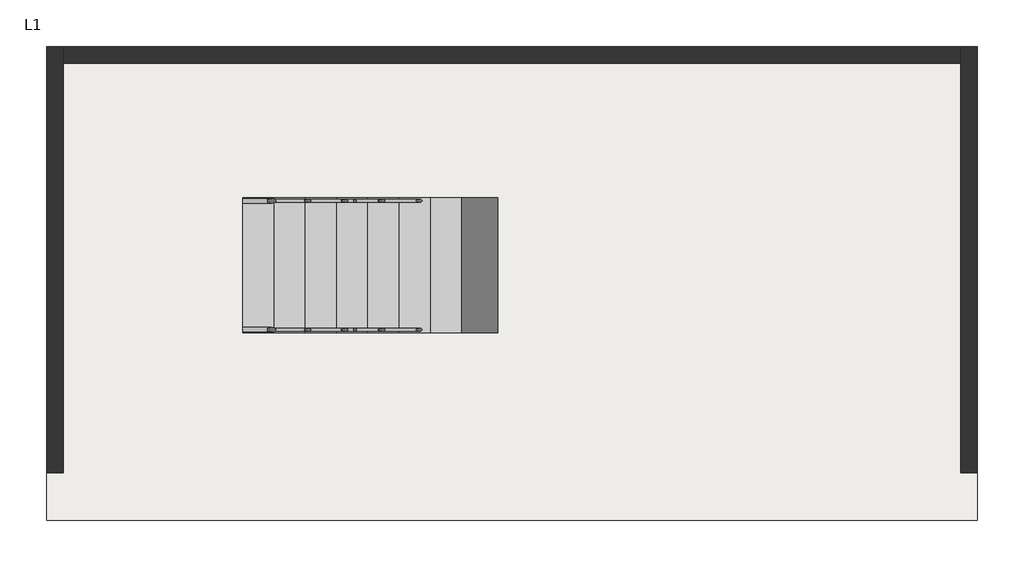
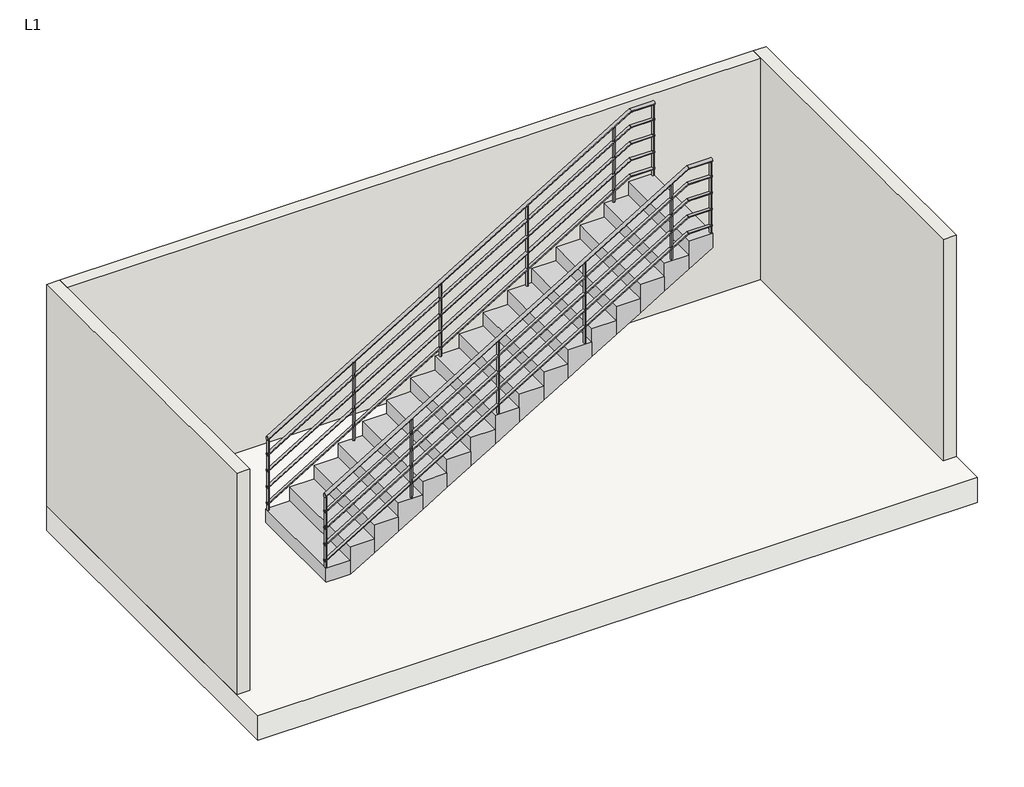
# One storey: 3 walls, 2 railings, 1 slab, 1 stair flight.
"""IFC4 building model written with IfcOpenShell, lengths in millimetres."""

from ifc_helpers import new_model, si_unit, point, frame, frame_2d, origin, origin_with_axes, place, context, project, spatial, polyline, circle_curve, ellipse_curve, trimmed, segment, composite_curve, outline, extrude, faceted_brep, element, save
from ifc_brep_helpers import plane_surface, cylinder_surface, advanced_brep

model = new_model("IFC4")

# Units and contexts
model_context = context("Model", 3, world=origin())
ifc_project = project(units=[si_unit("LENGTHUNIT", "METRE", prefix="MILLI")], contexts=[model_context])

# Site, building, storey
site = spatial("IfcSite", under=ifc_project)
building = spatial("IfcBuilding", under=site)
storey = spatial("IfcBuildingStorey", under=building, Name="L1", Elevation=0.0)

# Railings
placement = place(None, origin())
element("IfcRailing", 1, ObjectType="900mm Pipe", at=placement, inside=storey, context=model_context, shape_type="SolidModel", body=[
    advanced_brep(
    [(-6625.0, 1680.4, 1045.3762552), (-6625.0, 1720.4, 1045.3762552), (-2434.4220753, 1680.4, 3580.0), (-2434.4220753, 1720.4, 3580.0), (-2161.0, 1680.4, 3580.0), (-2161.0, 1720.4, 3580.0)],
    [
        (0, 1, ellipse_curve(frame((-6625.0, 1700.4, 1045.3762552), z_axis=(-1.0, 0.0, 0.0), x_axis=(0.0, 0.0, -1.0)), 23.3737448, 20.0)),
        (1, 0, ellipse_curve(frame((-6625.0, 1700.4, 1045.3762552), z_axis=(-1.0, 0.0, 0.0), x_axis=(0.0, 0.0, -1.0)), 23.3737448, 20.0)),
        (0, 2),
        (2, 3, ellipse_curve(frame((-2434.4220753, 1700.4, 3580.0), z_axis=(-0.9632395654633321, 0.0, -0.26864388979839315), x_axis=(0.2686438897983936, 0.0, -0.9632395654633319)), 20.7632667, 20.0)),
        (3, 1),
        (3, 2, ellipse_curve(frame((-2434.4220753, 1700.4, 3580.0), z_axis=(-0.9632395654633321, 0.0, -0.26864388979839315), x_axis=(0.2686438897983936, 0.0, -0.9632395654633319)), 20.7632667, 20.0)),
        (4, 5, circle_curve(frame((-2161.0, 1700.4, 3580.0), z_axis=(1.0, 0.0, 0.0), x_axis=(0.0, 1.0, 0.0)), 20.0)),
        (5, 4, circle_curve(frame((-2161.0, 1700.4, 3580.0), z_axis=(1.0, 0.0, 0.0), x_axis=(0.0, 1.0, 0.0)), 20.0)),
        (2, 4),
        (5, 3),
    ],
    [
        plane_surface(frame((-6625.0, 1700.4, 1068.75), z_axis=(-1.0, 0.0, 0.0), x_axis=(0.0, 1.0, 0.0))),
        cylinder_surface(frame((-6614.6492631, 1700.4, 1051.6367816), z_axis=(-0.8556609209479775, 0.0, -0.517536847347567), x_axis=(0.0, 1.0, 0.0)), 20.0),
        plane_surface(frame((-2161.0, 1700.4, 3600.0), z_axis=(1.0, 0.0, 0.0), x_axis=(0.0, 1.0, 0.0))),
        cylinder_surface(frame((-2440.0, 1700.4, 3580.0), z_axis=(-1.0, 0.0, 0.0), x_axis=(0.0, 1.0, 0.0)), 20.0),
    ],
    [
        (0, [[1, 2]]),
        (1, [[-1, 3, 4, 5]]),
        (1, [[-2, -5, 6, -3]]),
        (2, [[7, 8]]),
        (3, [[-4, 9, -8, 10]]),
        (3, [[-6, -10, -7, -9]]),
    ],
),
    advanced_brep(
    [(-6625.0, 1715.4, 851.2196914), (-6625.0, 1685.4, 851.2196914), (-2435.8165565, 1715.4, 3385.0), (-2435.8165565, 1685.4, 3385.0), (-2161.0, 1715.4, 3385.0), (-2161.0, 1685.4, 3385.0)],
    [
        (0, 1, ellipse_curve(frame((-6625.0, 1700.4, 851.2196914), z_axis=(-1.0, 0.0, 0.0), x_axis=(0.0, 0.0, -1.0)), 17.5303086, 15.0)),
        (1, 0, ellipse_curve(frame((-6625.0, 1700.4, 851.2196914), z_axis=(-1.0, 0.0, 0.0), x_axis=(0.0, 0.0, -1.0)), 17.5303086, 15.0)),
        (0, 2),
        (2, 3, ellipse_curve(frame((-2435.8165565, 1700.4, 3385.0), z_axis=(-0.9632395654633321, 0.0, -0.26864388979839315), x_axis=(0.2686438897983936, 0.0, -0.9632395654633319)), 15.57245, 15.0)),
        (3, 1),
        (3, 2, ellipse_curve(frame((-2435.8165565, 1700.4, 3385.0), z_axis=(-0.9632395654633321, 0.0, -0.26864388979839315), x_axis=(0.2686438897983936, 0.0, -0.9632395654633319)), 15.57245, 15.0)),
        (4, 5, circle_curve(frame((-2161.0, 1700.4, 3385.0), z_axis=(1.0, 0.0, 0.0), x_axis=(0.0, -1.0, 0.0)), 15.0)),
        (5, 4, circle_curve(frame((-2161.0, 1700.4, 3385.0), z_axis=(1.0, 0.0, 0.0), x_axis=(0.0, -1.0, 0.0)), 15.0)),
        (2, 4),
        (5, 3),
    ],
    [
        plane_surface(frame((-6625.0, 1700.4, 868.75), z_axis=(-1.0, 0.0, 0.0), x_axis=(0.0, 1.0, 0.0))),
        cylinder_surface(frame((-6617.2369473, 1700.4, 855.9150862), z_axis=(-0.8556609209479775, 0.0, -0.517536847347567), x_axis=(0.0, -1.0, 0.0)), 15.0),
        plane_surface(frame((-2161.0, 1700.4, 3400.0), z_axis=(1.0, 0.0, 0.0), x_axis=(0.0, 1.0, 0.0))),
        cylinder_surface(frame((-2440.0, 1700.4, 3385.0), z_axis=(-1.0, 0.0, 0.0), x_axis=(0.0, -1.0, 0.0)), 15.0),
    ],
    [
        (0, [[1, 2]]),
        (1, [[-1, 3, 4, 5]]),
        (1, [[-2, -5, 6, -3]]),
        (2, [[7, 8]]),
        (3, [[-4, 9, -8, 10]]),
        (3, [[-6, -10, -7, -9]]),
    ],
),
    advanced_brep(
    [(-6625.0, 1715.4, 651.2196914), (-6625.0, 1685.4, 651.2196914), (-2435.8165565, 1715.4, 3185.0), (-2435.8165565, 1685.4, 3185.0), (-2161.0, 1715.4, 3185.0), (-2161.0, 1685.4, 3185.0)],
    [
        (0, 1, ellipse_curve(frame((-6625.0, 1700.4, 651.2196914), z_axis=(-1.0, 0.0, 0.0), x_axis=(0.0, 0.0, -1.0)), 17.5303086, 15.0)),
        (1, 0, ellipse_curve(frame((-6625.0, 1700.4, 651.2196914), z_axis=(-1.0, 0.0, 0.0), x_axis=(0.0, 0.0, -1.0)), 17.5303086, 15.0)),
        (0, 2),
        (2, 3, ellipse_curve(frame((-2435.8165565, 1700.4, 3185.0), z_axis=(-0.9632395654633321, 0.0, -0.26864388979839315), x_axis=(0.2686438897983936, 0.0, -0.9632395654633319)), 15.57245, 15.0)),
        (3, 1),
        (3, 2, ellipse_curve(frame((-2435.8165565, 1700.4, 3185.0), z_axis=(-0.9632395654633321, 0.0, -0.26864388979839315), x_axis=(0.2686438897983936, 0.0, -0.9632395654633319)), 15.57245, 15.0)),
        (4, 5, circle_curve(frame((-2161.0, 1700.4, 3185.0), z_axis=(1.0, 0.0, 0.0), x_axis=(0.0, -1.0, 0.0)), 15.0)),
        (5, 4, circle_curve(frame((-2161.0, 1700.4, 3185.0), z_axis=(1.0, 0.0, 0.0), x_axis=(0.0, -1.0, 0.0)), 15.0)),
        (2, 4),
        (5, 3),
    ],
    [
        plane_surface(frame((-6625.0, 1700.4, 668.75), z_axis=(-1.0, 0.0, 0.0), x_axis=(0.0, 1.0, 0.0))),
        cylinder_surface(frame((-6617.2369473, 1700.4, 655.9150862), z_axis=(-0.8556609209479775, 0.0, -0.517536847347567), x_axis=(0.0, -1.0, 0.0)), 15.0),
        plane_surface(frame((-2161.0, 1700.4, 3200.0), z_axis=(1.0, 0.0, 0.0), x_axis=(0.0, 1.0, 0.0))),
        cylinder_surface(frame((-2440.0, 1700.4, 3185.0), z_axis=(-1.0, 0.0, 0.0), x_axis=(0.0, -1.0, 0.0)), 15.0),
    ],
    [
        (0, [[1, 2]]),
        (1, [[-1, 3, 4, 5]]),
        (1, [[-2, -5, 6, -3]]),
        (2, [[7, 8]]),
        (3, [[-4, 9, -8, 10]]),
        (3, [[-6, -10, -7, -9]]),
    ],
),
    advanced_brep(
    [(-6625.0, 1715.4, 451.2196914), (-6625.0, 1685.4, 451.2196914), (-2435.8165565, 1715.4, 2985.0), (-2435.8165565, 1685.4, 2985.0), (-2161.0, 1715.4, 2985.0), (-2161.0, 1685.4, 2985.0)],
    [
        (0, 1, ellipse_curve(frame((-6625.0, 1700.4, 451.2196914), z_axis=(-1.0, 0.0, 0.0), x_axis=(0.0, 0.0, -1.0)), 17.5303086, 15.0)),
        (1, 0, ellipse_curve(frame((-6625.0, 1700.4, 451.2196914), z_axis=(-1.0, 0.0, 0.0), x_axis=(0.0, 0.0, -1.0)), 17.5303086, 15.0)),
        (0, 2),
        (2, 3, ellipse_curve(frame((-2435.8165565, 1700.4, 2985.0), z_axis=(-0.9632395654633321, 0.0, -0.26864388979839315), x_axis=(0.2686438897983936, 0.0, -0.9632395654633319)), 15.57245, 15.0)),
        (3, 1),
        (3, 2, ellipse_curve(frame((-2435.8165565, 1700.4, 2985.0), z_axis=(-0.9632395654633321, 0.0, -0.26864388979839315), x_axis=(0.2686438897983936, 0.0, -0.9632395654633319)), 15.57245, 15.0)),
        (4, 5, circle_curve(frame((-2161.0, 1700.4, 2985.0), z_axis=(1.0, 0.0, 0.0), x_axis=(0.0, -1.0, 0.0)), 15.0)),
        (5, 4, circle_curve(frame((-2161.0, 1700.4, 2985.0), z_axis=(1.0, 0.0, 0.0), x_axis=(0.0, -1.0, 0.0)), 15.0)),
        (2, 4),
        (5, 3),
    ],
    [
        plane_surface(frame((-6625.0, 1700.4, 468.75), z_axis=(-1.0, 0.0, 0.0), x_axis=(0.0, 1.0, 0.0))),
        cylinder_surface(frame((-6617.2369473, 1700.4, 455.9150862), z_axis=(-0.8556609209479775, 0.0, -0.517536847347567), x_axis=(0.0, -1.0, 0.0)), 15.0),
        plane_surface(frame((-2161.0, 1700.4, 3000.0), z_axis=(1.0, 0.0, 0.0), x_axis=(0.0, 1.0, 0.0))),
        cylinder_surface(frame((-2440.0, 1700.4, 2985.0), z_axis=(-1.0, 0.0, 0.0), x_axis=(0.0, -1.0, 0.0)), 15.0),
    ],
    [
        (0, [[1, 2]]),
        (1, [[-1, 3, 4, 5]]),
        (1, [[-2, -5, 6, -3]]),
        (2, [[7, 8]]),
        (3, [[-4, 9, -8, 10]]),
        (3, [[-6, -10, -7, -9]]),
    ],
),
    advanced_brep(
    [(-6625.0, 1715.4, 251.2196914), (-6625.0, 1685.4, 251.2196914), (-2435.8165565, 1715.4, 2785.0), (-2435.8165565, 1685.4, 2785.0), (-2161.0, 1715.4, 2785.0), (-2161.0, 1685.4, 2785.0)],
    [
        (0, 1, ellipse_curve(frame((-6625.0, 1700.4, 251.2196914), z_axis=(-1.0, 0.0, 0.0), x_axis=(0.0, 0.0, -1.0)), 17.5303086, 15.0)),
        (1, 0, ellipse_curve(frame((-6625.0, 1700.4, 251.2196914), z_axis=(-1.0, 0.0, 0.0), x_axis=(0.0, 0.0, -1.0)), 17.5303086, 15.0)),
        (0, 2),
        (2, 3, ellipse_curve(frame((-2435.8165565, 1700.4, 2785.0), z_axis=(-0.9632395654633321, 0.0, -0.26864388979839315), x_axis=(0.2686438897983936, 0.0, -0.9632395654633319)), 15.57245, 15.0)),
        (3, 1),
        (3, 2, ellipse_curve(frame((-2435.8165565, 1700.4, 2785.0), z_axis=(-0.9632395654633321, 0.0, -0.26864388979839315), x_axis=(0.2686438897983936, 0.0, -0.9632395654633319)), 15.57245, 15.0)),
        (4, 5, circle_curve(frame((-2161.0, 1700.4, 2785.0), z_axis=(1.0, 0.0, 0.0), x_axis=(0.0, -1.0, 0.0)), 15.0)),
        (5, 4, circle_curve(frame((-2161.0, 1700.4, 2785.0), z_axis=(1.0, 0.0, 0.0), x_axis=(0.0, -1.0, 0.0)), 15.0)),
        (2, 4),
        (5, 3),
    ],
    [
        plane_surface(frame((-6625.0, 1700.4, 268.75), z_axis=(-1.0, 0.0, 0.0), x_axis=(0.0, 1.0, 0.0))),
        cylinder_surface(frame((-6617.2369473, 1700.4, 255.9150862), z_axis=(-0.8556609209479775, 0.0, -0.517536847347567), x_axis=(0.0, -1.0, 0.0)), 15.0),
        plane_surface(frame((-2161.0, 1700.4, 2800.0), z_axis=(1.0, 0.0, 0.0), x_axis=(0.0, 1.0, 0.0))),
        cylinder_surface(frame((-2440.0, 1700.4, 2785.0), z_axis=(-1.0, 0.0, 0.0), x_axis=(0.0, -1.0, 0.0)), 15.0),
    ],
    [
        (0, [[1, 2]]),
        (1, [[-1, 3, 4, 5]]),
        (1, [[-2, -5, 6, -3]]),
        (2, [[7, 8]]),
        (3, [[-4, 9, -8, 10]]),
        (3, [[-6, -10, -7, -9]]),
    ],
),
    advanced_brep(
    [(-2625.0, 1687.9, 3441.3573491), (-2625.0, 1687.9, 2531.25), (-2625.0, 1712.9, 2531.25), (-2625.0, 1712.9, 3441.3573491)],
    [
        (0, 1),
        (1, 2, circle_curve(frame((-2625.0, 1700.4, 2531.25), z_axis=(0.0, 0.0, 1.0), x_axis=(0.0, 1.0, 0.0)), 12.5)),
        (2, 3),
        (3, 0, ellipse_curve(frame((-2625.0, 1700.4, 3441.3573491), z_axis=(0.5175368473475664, 0.0, -0.8556609209479781), x_axis=(0.8556609209479781, 0.0, 0.517536847347566)), 14.6085905, 12.5)),
        (0, 3, ellipse_curve(frame((-2625.0, 1700.4, 3441.3573491), z_axis=(0.5175368473475664, 0.0, -0.8556609209479781), x_axis=(0.8556609209479781, 0.0, 0.517536847347566)), 14.6085905, 12.5)),
        (2, 1, circle_curve(frame((-2625.0, 1700.4, 2531.25), z_axis=(0.0, 0.0, 1.0), x_axis=(0.0, 1.0, 0.0)), 12.5)),
    ],
    [
        cylinder_surface(frame((-2625.0, 1700.4, 2431.25), z_axis=(0.0, 0.0, 1.0), x_axis=(0.0, 1.0, 0.0)), 12.5),
        plane_surface(frame((-2600.0, 1725.4, 3456.4783169), z_axis=(-0.5175368473475664, 0.0, 0.8556609209479781), x_axis=(0.0, -1.0, 0.0))),
        plane_surface(frame((-2650.0, 1725.4, 2531.25), z_axis=(0.0, 0.0, -1.0), x_axis=(0.0, -1.0, 0.0))),
    ],
    [
        (0, [[1, 2, 3, 4]]),
        (0, [[-1, 5, -3, 6]]),
        (1, [[-4, -5]]),
        (2, [[-2, -6]]),
    ],
),
    advanced_brep(
    [(-3625.0, 1687.9, 2836.5186394), (-3625.0, 1687.9, 1856.25), (-3625.0, 1712.9, 1856.25), (-3625.0, 1712.9, 2836.5186394)],
    [
        (0, 1),
        (1, 2, circle_curve(frame((-3625.0, 1700.4, 1856.25), z_axis=(0.0, 0.0, 1.0), x_axis=(0.0, 1.0, 0.0)), 12.5)),
        (2, 3),
        (3, 0, ellipse_curve(frame((-3625.0, 1700.4, 2836.5186394), z_axis=(0.5175368473475664, 0.0, -0.8556609209479781), x_axis=(0.8556609209479781, 0.0, 0.517536847347566)), 14.6085905, 12.5)),
        (0, 3, ellipse_curve(frame((-3625.0, 1700.4, 2836.5186394), z_axis=(0.5175368473475664, 0.0, -0.8556609209479781), x_axis=(0.8556609209479781, 0.0, 0.517536847347566)), 14.6085905, 12.5)),
        (2, 1, circle_curve(frame((-3625.0, 1700.4, 1856.25), z_axis=(0.0, 0.0, 1.0), x_axis=(0.0, 1.0, 0.0)), 12.5)),
    ],
    [
        cylinder_surface(frame((-3625.0, 1700.4, 1756.25), z_axis=(0.0, 0.0, 1.0), x_axis=(0.0, 1.0, 0.0)), 12.5),
        plane_surface(frame((-3600.0, 1725.4, 2851.6396072), z_axis=(-0.5175368473475664, 0.0, 0.8556609209479781), x_axis=(0.0, -1.0, 0.0))),
        plane_surface(frame((-3650.0, 1725.4, 1856.25), z_axis=(0.0, 0.0, -1.0), x_axis=(0.0, -1.0, 0.0))),
    ],
    [
        (0, [[1, 2, 3, 4]]),
        (0, [[-1, 5, -3, 6]]),
        (1, [[-4, -5]]),
        (2, [[-2, -6]]),
    ],
),
    advanced_brep(
    [(-4625.0, 1687.9, 2231.6799298), (-4625.0, 1687.9, 1350.0), (-4625.0, 1712.9, 1350.0), (-4625.0, 1712.9, 2231.6799298)],
    [
        (0, 1),
        (1, 2, circle_curve(frame((-4625.0, 1700.4, 1350.0), z_axis=(0.0, 0.0, 1.0), x_axis=(0.0, 1.0, 0.0)), 12.5)),
        (2, 3),
        (3, 0, ellipse_curve(frame((-4625.0, 1700.4, 2231.6799298), z_axis=(0.5175368473475664, 0.0, -0.8556609209479781), x_axis=(0.8556609209479781, 0.0, 0.517536847347566)), 14.6085905, 12.5)),
        (0, 3, ellipse_curve(frame((-4625.0, 1700.4, 2231.6799298), z_axis=(0.5175368473475664, 0.0, -0.8556609209479781), x_axis=(0.8556609209479781, 0.0, 0.517536847347566)), 14.6085905, 12.5)),
        (2, 1, circle_curve(frame((-4625.0, 1700.4, 1350.0), z_axis=(0.0, 0.0, 1.0), x_axis=(0.0, 1.0, 0.0)), 12.5)),
    ],
    [
        cylinder_surface(frame((-4625.0, 1700.4, 1250.0), z_axis=(0.0, 0.0, 1.0), x_axis=(0.0, 1.0, 0.0)), 12.5),
        plane_surface(frame((-4600.0, 1725.4, 2246.8008975), z_axis=(-0.5175368473475664, 0.0, 0.8556609209479781), x_axis=(0.0, -1.0, 0.0))),
        plane_surface(frame((-4650.0, 1725.4, 1350.0), z_axis=(0.0, 0.0, -1.0), x_axis=(0.0, -1.0, 0.0))),
    ],
    [
        (0, [[1, 2, 3, 4]]),
        (0, [[-1, 5, -3, 6]]),
        (1, [[-4, -5]]),
        (2, [[-2, -6]]),
    ],
),
    advanced_brep(
    [(-5625.0, 1687.9, 1626.8412201), (-5625.0, 1687.9, 675.0), (-5625.0, 1712.9, 675.0), (-5625.0, 1712.9, 1626.8412201)],
    [
        (0, 1),
        (1, 2, circle_curve(frame((-5625.0, 1700.4, 675.0), z_axis=(0.0, 0.0, 1.0), x_axis=(0.0, 1.0, 0.0)), 12.5)),
        (2, 3),
        (3, 0, ellipse_curve(frame((-5625.0, 1700.4, 1626.8412201), z_axis=(0.5175368473475664, 0.0, -0.8556609209479781), x_axis=(0.8556609209479781, 0.0, 0.517536847347566)), 14.6085905, 12.5)),
        (0, 3, ellipse_curve(frame((-5625.0, 1700.4, 1626.8412201), z_axis=(0.5175368473475664, 0.0, -0.8556609209479781), x_axis=(0.8556609209479781, 0.0, 0.517536847347566)), 14.6085905, 12.5)),
        (2, 1, circle_curve(frame((-5625.0, 1700.4, 675.0), z_axis=(0.0, 0.0, 1.0), x_axis=(0.0, 1.0, 0.0)), 12.5)),
    ],
    [
        cylinder_surface(frame((-5625.0, 1700.4, 575.0), z_axis=(0.0, 0.0, 1.0), x_axis=(0.0, 1.0, 0.0)), 12.5),
        plane_surface(frame((-5600.0, 1725.4, 1641.9621878), z_axis=(-0.5175368473475664, 0.0, 0.8556609209479781), x_axis=(0.0, -1.0, 0.0))),
        plane_surface(frame((-5650.0, 1725.4, 675.0), z_axis=(0.0, 0.0, -1.0), x_axis=(0.0, -1.0, 0.0))),
    ],
    [
        (0, [[1, 2, 3, 4]]),
        (0, [[-1, 5, -3, 6]]),
        (1, [[-4, -5]]),
        (2, [[-2, -6]]),
    ],
),
    extrude(outline(composite_curve([segment(trimmed(circle_curve(frame_2d((-2173.5, 1700.4)), 12.5), [point((-2173.5, 1712.9))], [point((-2173.5, 1687.9))], False, "CARTESIAN"), True, "CONTINUOUS"), segment(trimmed(circle_curve(frame_2d((-2173.5, 1700.4)), 12.5), [point((-2173.5, 1687.9))], [point((-2173.5, 1712.9))], False, "CARTESIAN"), True, "CONTINUOUS")], self_intersect=False)), frame((0.0, 0.0, 2700.0), z_axis=(0.0, 0.0, 1.0), x_axis=(1.0, 0.0, 0.0)), (0.0, 0.0, 1.0), 860.0),
    advanced_brep(
    [(-6612.5, 1687.9, 1029.5629943), (-6612.5, 1687.9, 168.75), (-6612.5, 1712.9, 168.75), (-6612.5, 1712.9, 1029.5629943)],
    [
        (0, 1),
        (1, 2, circle_curve(frame((-6612.5, 1700.4, 168.75), z_axis=(0.0, 0.0, 1.0), x_axis=(0.0, 1.0, 0.0)), 12.5)),
        (2, 3),
        (3, 0, ellipse_curve(frame((-6612.5, 1700.4, 1029.5629943), z_axis=(0.5175368473475664, 0.0, -0.8556609209479781), x_axis=(0.8556609209479781, 0.0, 0.517536847347566)), 14.6085905, 12.5)),
        (0, 3, ellipse_curve(frame((-6612.5, 1700.4, 1029.5629943), z_axis=(0.5175368473475664, 0.0, -0.8556609209479781), x_axis=(0.8556609209479781, 0.0, 0.517536847347566)), 14.6085905, 12.5)),
        (2, 1, circle_curve(frame((-6612.5, 1700.4, 168.75), z_axis=(0.0, 0.0, 1.0), x_axis=(0.0, 1.0, 0.0)), 12.5)),
    ],
    [
        cylinder_surface(frame((-6612.5, 1700.4, 68.75), z_axis=(0.0, 0.0, 1.0), x_axis=(0.0, 1.0, 0.0)), 12.5),
        plane_surface(frame((-6587.5, 1725.4, 1044.683962), z_axis=(-0.5175368473475664, 0.0, 0.8556609209479781), x_axis=(0.0, -1.0, 0.0))),
        plane_surface(frame((-6637.5, 1725.4, 168.75), z_axis=(0.0, 0.0, -1.0), x_axis=(0.0, -1.0, 0.0))),
    ],
    [
        (0, [[1, 2, 3, 4]]),
        (0, [[-1, 5, -3, 6]]),
        (1, [[-4, -5]]),
        (2, [[-2, -6]]),
    ],
),
])
element("IfcRailing", 2, ObjectType="900mm Pipe", at=placement, inside=storey, context=model_context, shape_type="SolidModel", body=[
    advanced_brep(
    [(-6625.0, 2829.6, 1045.3762552), (-6625.0, 2869.6, 1045.3762552), (-2434.4220753, 2829.6, 3580.0), (-2434.4220753, 2869.6, 3580.0), (-2161.0, 2829.6, 3580.0), (-2161.0, 2869.6, 3580.0)],
    [
        (0, 1, ellipse_curve(frame((-6625.0, 2849.6, 1045.3762552), z_axis=(-1.0, 0.0, 0.0), x_axis=(0.0, 0.0, -1.0)), 23.3737448, 20.0)),
        (1, 0, ellipse_curve(frame((-6625.0, 2849.6, 1045.3762552), z_axis=(-1.0, 0.0, 0.0), x_axis=(0.0, 0.0, -1.0)), 23.3737448, 20.0)),
        (0, 2),
        (2, 3, ellipse_curve(frame((-2434.4220753, 2849.6, 3580.0), z_axis=(-0.9632395654633321, 0.0, -0.2686438897983932), x_axis=(0.2686438897983936, 0.0, -0.963239565463332)), 20.7632667, 20.0)),
        (3, 1),
        (3, 2, ellipse_curve(frame((-2434.4220753, 2849.6, 3580.0), z_axis=(-0.9632395654633321, 0.0, -0.2686438897983932), x_axis=(0.2686438897983936, 0.0, -0.963239565463332)), 20.7632667, 20.0)),
        (4, 5, circle_curve(frame((-2161.0, 2849.6, 3580.0), z_axis=(1.0, 0.0, 0.0), x_axis=(0.0, 1.0, 0.0)), 20.0)),
        (5, 4, circle_curve(frame((-2161.0, 2849.6, 3580.0), z_axis=(1.0, 0.0, 0.0), x_axis=(0.0, 1.0, 0.0)), 20.0)),
        (2, 4),
        (5, 3),
    ],
    [
        plane_surface(frame((-6625.0, 2849.6, 1068.75), z_axis=(-1.0, 0.0, 0.0), x_axis=(0.0, 1.0, 0.0))),
        cylinder_surface(frame((-6614.6492631, 2849.6, 1051.6367816), z_axis=(-0.8556609209479775, 0.0, -0.5175368473475671), x_axis=(0.0, 1.0, 0.0)), 20.0),
        plane_surface(frame((-2161.0, 2849.6, 3600.0), z_axis=(1.0, 0.0, 0.0), x_axis=(0.0, 1.0, 0.0))),
        cylinder_surface(frame((-2440.0, 2849.6, 3580.0), z_axis=(-1.0, 0.0, 0.0), x_axis=(0.0, 1.0, 0.0)), 20.0),
    ],
    [
        (0, [[1, 2]]),
        (1, [[-1, 3, 4, 5]]),
        (1, [[-2, -5, 6, -3]]),
        (2, [[7, 8]]),
        (3, [[-4, 9, -8, 10]]),
        (3, [[-6, -10, -7, -9]]),
    ],
),
    advanced_brep(
    [(-6625.0, 2834.6, 851.2196914), (-6625.0, 2864.6, 851.2196914), (-2435.8165565, 2834.6, 3385.0), (-2435.8165565, 2864.6, 3385.0), (-2161.0, 2834.6, 3385.0), (-2161.0, 2864.6, 3385.0)],
    [
        (0, 1, ellipse_curve(frame((-6625.0, 2849.6, 851.2196914), z_axis=(-1.0, 0.0, 0.0), x_axis=(0.0, 0.0, -1.0)), 17.5303086, 15.0)),
        (1, 0, ellipse_curve(frame((-6625.0, 2849.6, 851.2196914), z_axis=(-1.0, 0.0, 0.0), x_axis=(0.0, 0.0, -1.0)), 17.5303086, 15.0)),
        (0, 2),
        (2, 3, ellipse_curve(frame((-2435.8165565, 2849.6, 3385.0), z_axis=(-0.9632395654633321, 0.0, -0.2686438897983932), x_axis=(0.2686438897983936, 0.0, -0.963239565463332)), 15.57245, 15.0)),
        (3, 1),
        (3, 2, ellipse_curve(frame((-2435.8165565, 2849.6, 3385.0), z_axis=(-0.9632395654633321, 0.0, -0.2686438897983932), x_axis=(0.2686438897983936, 0.0, -0.963239565463332)), 15.57245, 15.0)),
        (4, 5, circle_curve(frame((-2161.0, 2849.6, 3385.0), z_axis=(1.0, 0.0, 0.0), x_axis=(0.0, 1.0, 0.0)), 15.0)),
        (5, 4, circle_curve(frame((-2161.0, 2849.6, 3385.0), z_axis=(1.0, 0.0, 0.0), x_axis=(0.0, 1.0, 0.0)), 15.0)),
        (2, 4),
        (5, 3),
    ],
    [
        plane_surface(frame((-6625.0, 2849.6, 868.75), z_axis=(-1.0, 0.0, 0.0), x_axis=(0.0, 1.0, 0.0))),
        cylinder_surface(frame((-6617.2369473, 2849.6, 855.9150862), z_axis=(-0.8556609209479775, 0.0, -0.5175368473475671), x_axis=(0.0, 1.0, 0.0)), 15.0),
        plane_surface(frame((-2161.0, 2849.6, 3400.0), z_axis=(1.0, 0.0, 0.0), x_axis=(0.0, 1.0, 0.0))),
        cylinder_surface(frame((-2440.0, 2849.6, 3385.0), z_axis=(-1.0, 0.0, 0.0), x_axis=(0.0, 1.0, 0.0)), 15.0),
    ],
    [
        (0, [[1, 2]]),
        (1, [[-1, 3, 4, 5]]),
        (1, [[-2, -5, 6, -3]]),
        (2, [[7, 8]]),
        (3, [[-4, 9, -8, 10]]),
        (3, [[-6, -10, -7, -9]]),
    ],
),
    advanced_brep(
    [(-6625.0, 2834.6, 651.2196914), (-6625.0, 2864.6, 651.2196914), (-2435.8165565, 2834.6, 3185.0), (-2435.8165565, 2864.6, 3185.0), (-2161.0, 2834.6, 3185.0), (-2161.0, 2864.6, 3185.0)],
    [
        (0, 1, ellipse_curve(frame((-6625.0, 2849.6, 651.2196914), z_axis=(-1.0, 0.0, 0.0), x_axis=(0.0, 0.0, -1.0)), 17.5303086, 15.0)),
        (1, 0, ellipse_curve(frame((-6625.0, 2849.6, 651.2196914), z_axis=(-1.0, 0.0, 0.0), x_axis=(0.0, 0.0, -1.0)), 17.5303086, 15.0)),
        (0, 2),
        (2, 3, ellipse_curve(frame((-2435.8165565, 2849.6, 3185.0), z_axis=(-0.9632395654633321, 0.0, -0.2686438897983932), x_axis=(0.2686438897983936, 0.0, -0.963239565463332)), 15.57245, 15.0)),
        (3, 1),
        (3, 2, ellipse_curve(frame((-2435.8165565, 2849.6, 3185.0), z_axis=(-0.9632395654633321, 0.0, -0.2686438897983932), x_axis=(0.2686438897983936, 0.0, -0.963239565463332)), 15.57245, 15.0)),
        (4, 5, circle_curve(frame((-2161.0, 2849.6, 3185.0), z_axis=(1.0, 0.0, 0.0), x_axis=(0.0, 1.0, 0.0)), 15.0)),
        (5, 4, circle_curve(frame((-2161.0, 2849.6, 3185.0), z_axis=(1.0, 0.0, 0.0), x_axis=(0.0, 1.0, 0.0)), 15.0)),
        (2, 4),
        (5, 3),
    ],
    [
        plane_surface(frame((-6625.0, 2849.6, 668.75), z_axis=(-1.0, 0.0, 0.0), x_axis=(0.0, 1.0, 0.0))),
        cylinder_surface(frame((-6617.2369473, 2849.6, 655.9150862), z_axis=(-0.8556609209479775, 0.0, -0.5175368473475671), x_axis=(0.0, 1.0, 0.0)), 15.0),
        plane_surface(frame((-2161.0, 2849.6, 3200.0), z_axis=(1.0, 0.0, 0.0), x_axis=(0.0, 1.0, 0.0))),
        cylinder_surface(frame((-2440.0, 2849.6, 3185.0), z_axis=(-1.0, 0.0, 0.0), x_axis=(0.0, 1.0, 0.0)), 15.0),
    ],
    [
        (0, [[1, 2]]),
        (1, [[-1, 3, 4, 5]]),
        (1, [[-2, -5, 6, -3]]),
        (2, [[7, 8]]),
        (3, [[-4, 9, -8, 10]]),
        (3, [[-6, -10, -7, -9]]),
    ],
),
    advanced_brep(
    [(-6625.0, 2834.6, 451.2196914), (-6625.0, 2864.6, 451.2196914), (-2435.8165565, 2834.6, 2985.0), (-2435.8165565, 2864.6, 2985.0), (-2161.0, 2834.6, 2985.0), (-2161.0, 2864.6, 2985.0)],
    [
        (0, 1, ellipse_curve(frame((-6625.0, 2849.6, 451.2196914), z_axis=(-1.0, 0.0, 0.0), x_axis=(0.0, 0.0, -1.0)), 17.5303086, 15.0)),
        (1, 0, ellipse_curve(frame((-6625.0, 2849.6, 451.2196914), z_axis=(-1.0, 0.0, 0.0), x_axis=(0.0, 0.0, -1.0)), 17.5303086, 15.0)),
        (0, 2),
        (2, 3, ellipse_curve(frame((-2435.8165565, 2849.6, 2985.0), z_axis=(-0.9632395654633321, 0.0, -0.2686438897983932), x_axis=(0.2686438897983936, 0.0, -0.963239565463332)), 15.57245, 15.0)),
        (3, 1),
        (3, 2, ellipse_curve(frame((-2435.8165565, 2849.6, 2985.0), z_axis=(-0.9632395654633321, 0.0, -0.2686438897983932), x_axis=(0.2686438897983936, 0.0, -0.963239565463332)), 15.57245, 15.0)),
        (4, 5, circle_curve(frame((-2161.0, 2849.6, 2985.0), z_axis=(1.0, 0.0, 0.0), x_axis=(0.0, 1.0, 0.0)), 15.0)),
        (5, 4, circle_curve(frame((-2161.0, 2849.6, 2985.0), z_axis=(1.0, 0.0, 0.0), x_axis=(0.0, 1.0, 0.0)), 15.0)),
        (2, 4),
        (5, 3),
    ],
    [
        plane_surface(frame((-6625.0, 2849.6, 468.75), z_axis=(-1.0, 0.0, 0.0), x_axis=(0.0, 1.0, 0.0))),
        cylinder_surface(frame((-6617.2369473, 2849.6, 455.9150862), z_axis=(-0.8556609209479775, 0.0, -0.5175368473475671), x_axis=(0.0, 1.0, 0.0)), 15.0),
        plane_surface(frame((-2161.0, 2849.6, 3000.0), z_axis=(1.0, 0.0, 0.0), x_axis=(0.0, 1.0, 0.0))),
        cylinder_surface(frame((-2440.0, 2849.6, 2985.0), z_axis=(-1.0, 0.0, 0.0), x_axis=(0.0, 1.0, 0.0)), 15.0),
    ],
    [
        (0, [[1, 2]]),
        (1, [[-1, 3, 4, 5]]),
        (1, [[-2, -5, 6, -3]]),
        (2, [[7, 8]]),
        (3, [[-4, 9, -8, 10]]),
        (3, [[-6, -10, -7, -9]]),
    ],
),
    advanced_brep(
    [(-6625.0, 2834.6, 251.2196914), (-6625.0, 2864.6, 251.2196914), (-2435.8165565, 2834.6, 2785.0), (-2435.8165565, 2864.6, 2785.0), (-2161.0, 2834.6, 2785.0), (-2161.0, 2864.6, 2785.0)],
    [
        (0, 1, ellipse_curve(frame((-6625.0, 2849.6, 251.2196914), z_axis=(-1.0, 0.0, 0.0), x_axis=(0.0, 0.0, -1.0)), 17.5303086, 15.0)),
        (1, 0, ellipse_curve(frame((-6625.0, 2849.6, 251.2196914), z_axis=(-1.0, 0.0, 0.0), x_axis=(0.0, 0.0, -1.0)), 17.5303086, 15.0)),
        (0, 2),
        (2, 3, ellipse_curve(frame((-2435.8165565, 2849.6, 2785.0), z_axis=(-0.9632395654633321, 0.0, -0.2686438897983932), x_axis=(0.2686438897983936, 0.0, -0.963239565463332)), 15.57245, 15.0)),
        (3, 1),
        (3, 2, ellipse_curve(frame((-2435.8165565, 2849.6, 2785.0), z_axis=(-0.9632395654633321, 0.0, -0.2686438897983932), x_axis=(0.2686438897983936, 0.0, -0.963239565463332)), 15.57245, 15.0)),
        (4, 5, circle_curve(frame((-2161.0, 2849.6, 2785.0), z_axis=(1.0, 0.0, 0.0), x_axis=(0.0, 1.0, 0.0)), 15.0)),
        (5, 4, circle_curve(frame((-2161.0, 2849.6, 2785.0), z_axis=(1.0, 0.0, 0.0), x_axis=(0.0, 1.0, 0.0)), 15.0)),
        (2, 4),
        (5, 3),
    ],
    [
        plane_surface(frame((-6625.0, 2849.6, 268.75), z_axis=(-1.0, 0.0, 0.0), x_axis=(0.0, 1.0, 0.0))),
        cylinder_surface(frame((-6617.2369473, 2849.6, 255.9150862), z_axis=(-0.8556609209479775, 0.0, -0.5175368473475671), x_axis=(0.0, 1.0, 0.0)), 15.0),
        plane_surface(frame((-2161.0, 2849.6, 2800.0), z_axis=(1.0, 0.0, 0.0), x_axis=(0.0, 1.0, 0.0))),
        cylinder_surface(frame((-2440.0, 2849.6, 2785.0), z_axis=(-1.0, 0.0, 0.0), x_axis=(0.0, 1.0, 0.0)), 15.0),
    ],
    [
        (0, [[1, 2]]),
        (1, [[-1, 3, 4, 5]]),
        (1, [[-2, -5, 6, -3]]),
        (2, [[7, 8]]),
        (3, [[-4, 9, -8, 10]]),
        (3, [[-6, -10, -7, -9]]),
    ],
),
    advanced_brep(
    [(-2625.0, 2862.1, 3441.3573491), (-2625.0, 2837.1, 3441.3573491), (-2625.0, 2837.1, 2531.25), (-2625.0, 2862.1, 2531.25)],
    [
        (0, 1, ellipse_curve(frame((-2625.0, 2849.6, 3441.3573491), z_axis=(0.5175368473475664, 0.0, -0.8556609209479781), x_axis=(0.8556609209479781, 0.0, 0.517536847347566)), 14.6085905, 12.5)),
        (1, 2),
        (2, 3, circle_curve(frame((-2625.0, 2849.6, 2531.25), z_axis=(0.0, 0.0, 1.0), x_axis=(0.0, -1.0, 0.0)), 12.5)),
        (3, 0),
        (3, 2, circle_curve(frame((-2625.0, 2849.6, 2531.25), z_axis=(0.0, 0.0, 1.0), x_axis=(0.0, -1.0, 0.0)), 12.5)),
        (1, 0, ellipse_curve(frame((-2625.0, 2849.6, 3441.3573491), z_axis=(0.5175368473475664, 0.0, -0.8556609209479781), x_axis=(0.8556609209479781, 0.0, 0.517536847347566)), 14.6085905, 12.5)),
    ],
    [
        cylinder_surface(frame((-2625.0, 2849.6, 2431.25), z_axis=(0.0, 0.0, 1.0), x_axis=(0.0, -1.0, 0.0)), 12.5),
        plane_surface(frame((-2600.0, 2824.6, 3456.4783169), z_axis=(-0.5175368473475664, 0.0, 0.8556609209479781), x_axis=(0.0, 1.0, 0.0))),
        plane_surface(frame((-2650.0, 2824.6, 2531.25), z_axis=(0.0, 0.0, -1.0), x_axis=(0.0, 1.0, 0.0))),
    ],
    [
        (0, [[1, 2, 3, 4]]),
        (0, [[5, -2, 6, -4]]),
        (1, [[-6, -1]]),
        (2, [[-5, -3]]),
    ],
),
    advanced_brep(
    [(-3625.0, 2862.1, 2836.5186394), (-3625.0, 2837.1, 2836.5186394), (-3625.0, 2837.1, 1856.25), (-3625.0, 2862.1, 1856.25)],
    [
        (0, 1, ellipse_curve(frame((-3625.0, 2849.6, 2836.5186394), z_axis=(0.5175368473475664, 0.0, -0.8556609209479781), x_axis=(0.8556609209479781, 0.0, 0.517536847347566)), 14.6085905, 12.5)),
        (1, 2),
        (2, 3, circle_curve(frame((-3625.0, 2849.6, 1856.25), z_axis=(0.0, 0.0, 1.0), x_axis=(0.0, -1.0, 0.0)), 12.5)),
        (3, 0),
        (3, 2, circle_curve(frame((-3625.0, 2849.6, 1856.25), z_axis=(0.0, 0.0, 1.0), x_axis=(0.0, -1.0, 0.0)), 12.5)),
        (1, 0, ellipse_curve(frame((-3625.0, 2849.6, 2836.5186394), z_axis=(0.5175368473475664, 0.0, -0.8556609209479781), x_axis=(0.8556609209479781, 0.0, 0.517536847347566)), 14.6085905, 12.5)),
    ],
    [
        cylinder_surface(frame((-3625.0, 2849.6, 1756.25), z_axis=(0.0, 0.0, 1.0), x_axis=(0.0, -1.0, 0.0)), 12.5),
        plane_surface(frame((-3600.0, 2824.6, 2851.6396072), z_axis=(-0.5175368473475664, 0.0, 0.8556609209479781), x_axis=(0.0, 1.0, 0.0))),
        plane_surface(frame((-3650.0, 2824.6, 1856.25), z_axis=(0.0, 0.0, -1.0), x_axis=(0.0, 1.0, 0.0))),
    ],
    [
        (0, [[1, 2, 3, 4]]),
        (0, [[5, -2, 6, -4]]),
        (1, [[-6, -1]]),
        (2, [[-5, -3]]),
    ],
),
    advanced_brep(
    [(-4625.0, 2862.1, 2231.6799298), (-4625.0, 2837.1, 2231.6799298), (-4625.0, 2837.1, 1350.0), (-4625.0, 2862.1, 1350.0)],
    [
        (0, 1, ellipse_curve(frame((-4625.0, 2849.6, 2231.6799298), z_axis=(0.5175368473475664, 0.0, -0.8556609209479781), x_axis=(0.8556609209479781, 0.0, 0.517536847347566)), 14.6085905, 12.5)),
        (1, 2),
        (2, 3, circle_curve(frame((-4625.0, 2849.6, 1350.0), z_axis=(0.0, 0.0, 1.0), x_axis=(0.0, -1.0, 0.0)), 12.5)),
        (3, 0),
        (3, 2, circle_curve(frame((-4625.0, 2849.6, 1350.0), z_axis=(0.0, 0.0, 1.0), x_axis=(0.0, -1.0, 0.0)), 12.5)),
        (1, 0, ellipse_curve(frame((-4625.0, 2849.6, 2231.6799298), z_axis=(0.5175368473475664, 0.0, -0.8556609209479781), x_axis=(0.8556609209479781, 0.0, 0.517536847347566)), 14.6085905, 12.5)),
    ],
    [
        cylinder_surface(frame((-4625.0, 2849.6, 1250.0), z_axis=(0.0, 0.0, 1.0), x_axis=(0.0, -1.0, 0.0)), 12.5),
        plane_surface(frame((-4600.0, 2824.6, 2246.8008975), z_axis=(-0.5175368473475664, 0.0, 0.8556609209479781), x_axis=(0.0, 1.0, 0.0))),
        plane_surface(frame((-4650.0, 2824.6, 1350.0), z_axis=(0.0, 0.0, -1.0), x_axis=(0.0, 1.0, 0.0))),
    ],
    [
        (0, [[1, 2, 3, 4]]),
        (0, [[5, -2, 6, -4]]),
        (1, [[-6, -1]]),
        (2, [[-5, -3]]),
    ],
),
    advanced_brep(
    [(-5625.0, 2862.1, 1626.8412201), (-5625.0, 2837.1, 1626.8412201), (-5625.0, 2837.1, 675.0), (-5625.0, 2862.1, 675.0)],
    [
        (0, 1, ellipse_curve(frame((-5625.0, 2849.6, 1626.8412201), z_axis=(0.5175368473475664, 0.0, -0.8556609209479781), x_axis=(0.8556609209479781, 0.0, 0.517536847347566)), 14.6085905, 12.5)),
        (1, 2),
        (2, 3, circle_curve(frame((-5625.0, 2849.6, 675.0), z_axis=(0.0, 0.0, 1.0), x_axis=(0.0, -1.0, 0.0)), 12.5)),
        (3, 0),
        (3, 2, circle_curve(frame((-5625.0, 2849.6, 675.0), z_axis=(0.0, 0.0, 1.0), x_axis=(0.0, -1.0, 0.0)), 12.5)),
        (1, 0, ellipse_curve(frame((-5625.0, 2849.6, 1626.8412201), z_axis=(0.5175368473475664, 0.0, -0.8556609209479781), x_axis=(0.8556609209479781, 0.0, 0.517536847347566)), 14.6085905, 12.5)),
    ],
    [
        cylinder_surface(frame((-5625.0, 2849.6, 575.0), z_axis=(0.0, 0.0, 1.0), x_axis=(0.0, -1.0, 0.0)), 12.5),
        plane_surface(frame((-5600.0, 2824.6, 1641.9621878), z_axis=(-0.5175368473475664, 0.0, 0.8556609209479781), x_axis=(0.0, 1.0, 0.0))),
        plane_surface(frame((-5650.0, 2824.6, 675.0), z_axis=(0.0, 0.0, -1.0), x_axis=(0.0, 1.0, 0.0))),
    ],
    [
        (0, [[1, 2, 3, 4]]),
        (0, [[5, -2, 6, -4]]),
        (1, [[-6, -1]]),
        (2, [[-5, -3]]),
    ],
),
    extrude(outline(composite_curve([segment(trimmed(circle_curve(frame_2d((-2173.5, 2849.6)), 12.5), [point((-2173.5, 2837.1))], [point((-2173.5, 2862.1))], False, "CARTESIAN"), True, "CONTINUOUS"), segment(trimmed(circle_curve(frame_2d((-2173.5, 2849.6)), 12.5), [point((-2173.5, 2862.1))], [point((-2173.5, 2837.1))], False, "CARTESIAN"), True, "CONTINUOUS")], self_intersect=False)), frame((0.0, 0.0, 2700.0), z_axis=(0.0, 0.0, 1.0), x_axis=(1.0, 0.0, 0.0)), (0.0, 0.0, 1.0), 860.0),
    advanced_brep(
    [(-6612.5, 2862.1, 1029.5629943), (-6612.5, 2837.1, 1029.5629943), (-6612.5, 2837.1, 168.75), (-6612.5, 2862.1, 168.75)],
    [
        (0, 1, ellipse_curve(frame((-6612.5, 2849.6, 1029.5629943), z_axis=(0.5175368473475664, 0.0, -0.8556609209479781), x_axis=(0.8556609209479781, 0.0, 0.517536847347566)), 14.6085905, 12.5)),
        (1, 2),
        (2, 3, circle_curve(frame((-6612.5, 2849.6, 168.75), z_axis=(0.0, 0.0, 1.0), x_axis=(0.0, -1.0, 0.0)), 12.5)),
        (3, 0),
        (3, 2, circle_curve(frame((-6612.5, 2849.6, 168.75), z_axis=(0.0, 0.0, 1.0), x_axis=(0.0, -1.0, 0.0)), 12.5)),
        (1, 0, ellipse_curve(frame((-6612.5, 2849.6, 1029.5629943), z_axis=(0.5175368473475664, 0.0, -0.8556609209479781), x_axis=(0.8556609209479781, 0.0, 0.517536847347566)), 14.6085905, 12.5)),
    ],
    [
        cylinder_surface(frame((-6612.5, 2849.6, 68.75), z_axis=(0.0, 0.0, 1.0), x_axis=(0.0, -1.0, 0.0)), 12.5),
        plane_surface(frame((-6587.5, 2824.6, 1044.683962), z_axis=(-0.5175368473475664, 0.0, 0.8556609209479781), x_axis=(0.0, 1.0, 0.0))),
        plane_surface(frame((-6637.5, 2824.6, 168.75), z_axis=(0.0, 0.0, -1.0), x_axis=(0.0, 1.0, 0.0))),
    ],
    [
        (0, [[1, 2, 3, 4]]),
        (0, [[5, -2, 6, -4]]),
        (1, [[-6, -1]]),
        (2, [[-5, -3]]),
    ],
),
])

# Slab
element("IfcSlab", 3, ObjectType="Generic 300mm", at=placement, inside=storey, context=model_context, shape_type="SweptSolid", body=[
    extrude(outline(polyline([(-75.0, 4225.0), (-75.0, 0.0), (-8375.0, 0.0), (-8375.0, 4225.0), (-75.0, 4225.0)])), frame((0.0, 0.0, -300.0), z_axis=(0.0, 0.0, 1.0), x_axis=(1.0, 0.0, 0.0)), (0.0, 0.0, 1.0), 300.0),
])

# Stair flight
element("IfcStairFlight", 4, ObjectType="M_Monolithic Run", at=placement, inside=storey, context=model_context, shape_type="Brep", body=[
    faceted_brep([(-6346.0, 2875.0, 168.75), (-6625.0, 2875.0, 168.75), (-6625.0, 1675.0, 168.75), (-6346.0, 1675.0, 168.75), (-6346.0, 2875.0, 0.0), (-6625.0, 2875.0, 0.0), (-6625.0, 1675.0, 0.0), (-6346.0, 1675.0, 0.0), (-6067.0, 2875.0, 337.5), (-6346.0, 2875.0, 337.5), (-6346.0, 1675.0, 337.5), (-6067.0, 1675.0, 337.5), (-6067.0, 2875.0, 162.196914), (-6335.1655645, 2875.0, 0.0), (-6335.1655645, 1675.0, 0.0), (-6067.0, 1675.0, 162.196914), (-5788.0, 2875.0, 506.25), (-6067.0, 2875.0, 506.25), (-6067.0, 1675.0, 506.25), (-5788.0, 1675.0, 506.25), (-5788.0, 2875.0, 330.946914), (-5788.0, 1675.0, 330.946914), (-5509.0, 2875.0, 675.0), (-5788.0, 2875.0, 675.0), (-5788.0, 1675.0, 675.0), (-5509.0, 1675.0, 675.0), (-5509.0, 2875.0, 499.696914), (-5509.0, 1675.0, 499.696914), (-5230.0, 2875.0, 843.75), (-5509.0, 2875.0, 843.75), (-5509.0, 1675.0, 843.75), (-5230.0, 1675.0, 843.75), (-5230.0, 2875.0, 668.446914), (-5230.0, 1675.0, 668.446914), (-4951.0, 2875.0, 1012.5), (-5230.0, 2875.0, 1012.5), (-5230.0, 1675.0, 1012.5), (-4951.0, 1675.0, 1012.5), (-4951.0, 2875.0, 837.196914), (-4951.0, 1675.0, 837.196914), (-4672.0, 2875.0, 1181.25), (-4951.0, 2875.0, 1181.25), (-4951.0, 1675.0, 1181.25), (-4672.0, 1675.0, 1181.25), (-4672.0, 2875.0, 1005.946914), (-4672.0, 1675.0, 1005.946914), (-4393.0, 2875.0, 1350.0), (-4672.0, 2875.0, 1350.0), (-4672.0, 1675.0, 1350.0), (-4393.0, 1675.0, 1350.0), (-4393.0, 2875.0, 1174.696914), (-4393.0, 1675.0, 1174.696914), (-4114.0, 2875.0, 1518.75), (-4393.0, 2875.0, 1518.75), (-4393.0, 1675.0, 1518.75), (-4114.0, 1675.0, 1518.75), (-4114.0, 2875.0, 1343.446914), (-4114.0, 1675.0, 1343.446914), (-3835.0, 2875.0, 1687.5), (-4114.0, 2875.0, 1687.5), (-4114.0, 1675.0, 1687.5), (-3835.0, 1675.0, 1687.5), (-3835.0, 2875.0, 1512.196914), (-3835.0, 1675.0, 1512.196914), (-3556.0, 2875.0, 1856.25), (-3835.0, 2875.0, 1856.25), (-3835.0, 1675.0, 1856.25), (-3556.0, 1675.0, 1856.25), (-3556.0, 2875.0, 1680.946914), (-3556.0, 1675.0, 1680.946914), (-3277.0, 2875.0, 2025.0), (-3556.0, 2875.0, 2025.0), (-3556.0, 1675.0, 2025.0), (-3277.0, 1675.0, 2025.0), (-3277.0, 2875.0, 1849.696914), (-3277.0, 1675.0, 1849.696914), (-2998.0, 2875.0, 2193.75), (-3277.0, 2875.0, 2193.75), (-3277.0, 1675.0, 2193.75), (-2998.0, 1675.0, 2193.75), (-2998.0, 2875.0, 2018.446914), (-2998.0, 1675.0, 2018.446914), (-2719.0, 2875.0, 2362.5), (-2998.0, 2875.0, 2362.5), (-2998.0, 1675.0, 2362.5), (-2719.0, 1675.0, 2362.5), (-2719.0, 2875.0, 2187.196914), (-2719.0, 1675.0, 2187.196914), (-2440.0, 2875.0, 2531.25), (-2719.0, 2875.0, 2531.25), (-2719.0, 1675.0, 2531.25), (-2440.0, 1675.0, 2531.25), (-2440.0, 2875.0, 2355.946914), (-2440.0, 1675.0, 2355.946914), (-2161.0, 2875.0, 2700.0), (-2440.0, 2875.0, 2700.0), (-2440.0, 1675.0, 2700.0), (-2161.0, 1675.0, 2700.0), (-2161.0, 2875.0, 2524.696914), (-2161.0, 1675.0, 2524.696914)], [[[0, 1, 2, 3]], [[1, 0, 4, 5]], [[2, 1, 5, 6]], [[3, 2, 6, 7]], [[8, 9, 10, 11]], [[4, 0, 9, 8, 12, 13]], [[0, 3, 10, 9]], [[3, 7, 14, 15, 11, 10]], [[16, 17, 18, 19]], [[17, 16, 20, 12, 8]], [[8, 11, 18, 17]], [[19, 18, 11, 15, 21]], [[22, 23, 24, 25]], [[23, 22, 26, 20, 16]], [[16, 19, 24, 23]], [[25, 24, 19, 21, 27]], [[28, 29, 30, 31]], [[29, 28, 32, 26, 22]], [[22, 25, 30, 29]], [[31, 30, 25, 27, 33]], [[34, 35, 36, 37]], [[35, 34, 38, 32, 28]], [[28, 31, 36, 35]], [[37, 36, 31, 33, 39]], [[40, 41, 42, 43]], [[41, 40, 44, 38, 34]], [[34, 37, 42, 41]], [[43, 42, 37, 39, 45]], [[46, 47, 48, 49]], [[47, 46, 50, 44, 40]], [[40, 43, 48, 47]], [[49, 48, 43, 45, 51]], [[52, 53, 54, 55]], [[53, 52, 56, 50, 46]], [[46, 49, 54, 53]], [[55, 54, 49, 51, 57]], [[58, 59, 60, 61]], [[59, 58, 62, 56, 52]], [[52, 55, 60, 59]], [[61, 60, 55, 57, 63]], [[64, 65, 66, 67]], [[65, 64, 68, 62, 58]], [[58, 61, 66, 65]], [[67, 66, 61, 63, 69]], [[70, 71, 72, 73]], [[71, 70, 74, 68, 64]], [[64, 67, 72, 71]], [[73, 72, 67, 69, 75]], [[76, 77, 78, 79]], [[77, 76, 80, 74, 70]], [[70, 73, 78, 77]], [[79, 78, 73, 75, 81]], [[82, 83, 84, 85]], [[83, 82, 86, 80, 76]], [[76, 79, 84, 83]], [[85, 84, 79, 81, 87]], [[88, 89, 90, 91]], [[89, 88, 92, 86, 82]], [[82, 85, 90, 89]], [[91, 90, 85, 87, 93]], [[94, 95, 96, 97]], [[95, 94, 98, 92, 88]], [[88, 91, 96, 95]], [[97, 96, 91, 93, 99]], [[94, 97, 99, 98]], [[5, 4, 13, 14, 7, 6]], [[14, 13, 12, 20, 26, 32, 38, 44, 50, 56, 62, 68, 74, 80, 86, 92, 98, 99, 93, 87, 81, 75, 69, 63, 57, 51, 45, 39, 33, 27, 21, 15]]]),
])

# Walls
element("IfcWall", 5, ObjectType="Generic - 150mm", at=placement, inside=storey, context=model_context, shape_type="Brep", body=[
    faceted_brep([(-75.0, 425.0, 0.0), (-75.0, 4225.0, 0.0), (-75.0, 4225.0, 2700.0), (-75.0, 425.0, 2700.0), (-225.0, 425.0, 0.0), (-225.0, 425.0, 2700.0), (-225.0, 4075.0, 2700.0), (-225.0, 4225.0, 2700.0), (-225.0, 4225.0, 0.0), (-225.0, 4075.0, 0.0)], [[[0, 1, 2, 3]], [[4, 5, 6, 7, 8, 9]], [[1, 0, 4, 9, 8]], [[3, 2, 7, 6, 5]], [[0, 3, 5, 4]], [[2, 1, 8, 7]]]),
])
element("IfcWall", 6, ObjectType="Generic - 150mm", at=placement, inside=storey, context=model_context, shape_type="Brep", body=[
    faceted_brep([(-8375.0, 4225.0, 0.0), (-8375.0, 425.0, 0.0), (-8375.0, 425.0, 2700.0), (-8375.0, 4225.0, 2700.0), (-8225.0, 4225.0, 0.0), (-8225.0, 4225.0, 2700.0), (-8225.0, 4075.0, 2700.0), (-8225.0, 425.0, 2700.0), (-8225.0, 425.0, 0.0), (-8225.0, 4075.0, 0.0)], [[[0, 1, 2, 3]], [[4, 5, 6, 7, 8, 9]], [[1, 0, 4, 9, 8]], [[2, 1, 8, 7]], [[3, 2, 7, 6, 5]], [[0, 3, 5, 4]]]),
])
element("IfcWall", 7, ObjectType="Generic - 150mm", at=placement, inside=storey, context=model_context, shape_type="SweptSolid", body=[
    extrude(outline(polyline([(-225.0, 4075.0), (-8225.0, 4075.0), (-8225.0, 4225.0), (-225.0, 4225.0), (-225.0, 4075.0)])), origin_with_axes(), (0.0, 0.0, 1.0), 2700.0),
])

save(model, "model.ifc")

# Revit data of these elements
# Project information
#   Название организации = "Organization Name"
#   Описание организации = "Organization Description"
#   Наименование здания = "Building Name"
#   Дата утверждения проекта = "Issue Date"
#   Статус проекта = "Project Status"
#   Заказчик = "Client Name"
#   Адрес проекта = "Enter address here\nAddress Line 2"
#   Наименование проекта = "Project Name"
#   Номер проекта = "Project Number"
# Type "900mm Pipe"
#   built-in parameter 1008612 = 0.019685 (stored number, unit not read)
#   built-in parameter 1008611 = 0.0984252 (stored number, unit not read)
#   built-in parameter 1008609 = 3.28084 (stored number, unit not read)
#   built-in parameter 1008604 = 0.19685 (stored number, unit not read)
#   built-in parameter 1008603 = 0.164042 (stored number, unit not read)
#   Railing Height = 900 mm
#   built-in parameter 1008630 = 2
#   built-in parameter 1008610 = 1
#   built-in parameter 1008605 = 1
#   built-in parameter 1008618 = M_Baluster - Round : 25mm
# Type "Generic 300mm"
#   Description = "Generic Floor (Material By Category), 300mm thick"
#   Function = 0
#   Layers, outside or top first: 300 mm no material (function 1)
# Type "Generic - 150mm"
#   Description = "Generic Wall (Material By Category), 150mm thick"
#   Type Mark = "G04"
#   Layers, outside or top first: 150 mm no material (function 1)
# Elements 1, 2 (IfcRailing, "900mm Pipe")
#   Phase Created = New Construction
# Element 3 (IfcSlab, "Generic 300mm")
#   Height Offset From Level = 0 mm
#   Phase Created = New Construction
#   Materials on its faces: "Default Floor"
# Element 4 (IfcStairFlight, "M_Monolithic Run")
#   Phase Created = New Construction
# Elements 5, 6, 7 (IfcWall, "Generic - 150mm")
#   Top Offset = 0 mm
#   Base Offset = 0 mm
#   Unconnected Height = 2700 mm
#   wall height = 2700 mm
#   Phase Created = New Construction
#   Base Constraint = L1
#   Materials on its faces: "Default Wall"
# Materials
#   "Default Floor": class "Miscellaneous", colour RGB 128 128 128, transparency 0, Cost = 0
#   "Default Wall": class "Miscellaneous", colour RGB 192 192 192, transparency 0, Cost = 0
